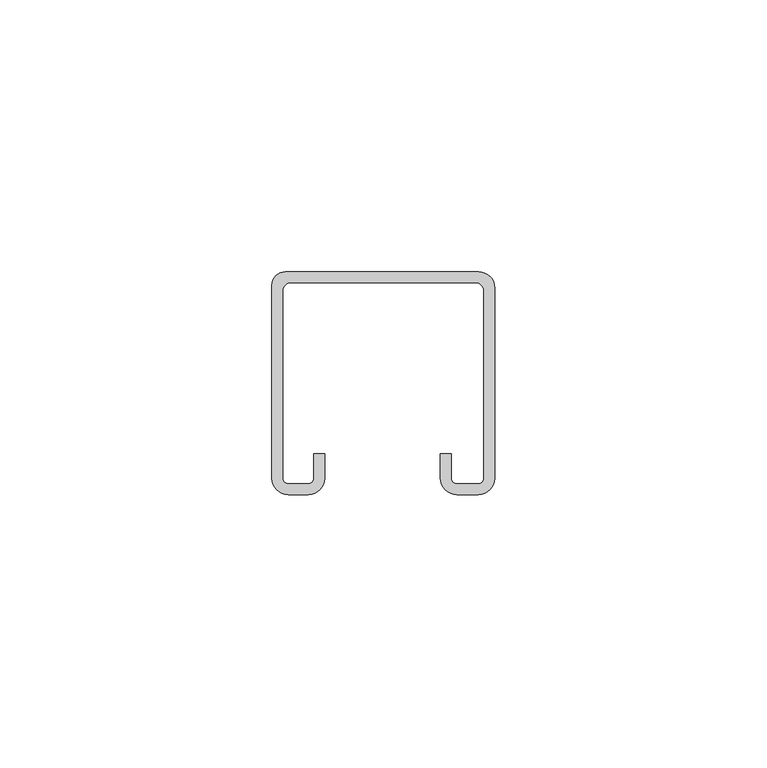
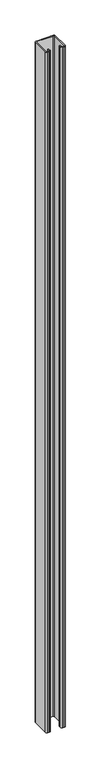
"""IFC4 building model written with IfcOpenShell, lengths in millimetres: proxy geometry, TN_Профиль монтажный : Профиль монтажный 41х41x2,0-3000."""

from ifc_helpers import new_model, si_unit, point, frame_2d, origin, origin_with_axes, place, context, project, spatial, polyline, circle_curve, trimmed, segment, composite_curve, outline, extrude, source, transform, mapped, element, save


def generic_models_c49aae80(model_context):
    return source(origin(), model_context, "Body", "SweptSolid", [
        extrude(outline(composite_curve([segment(polyline([(20.7157599, -2.9315199), (20.7157599, -38.0)]), True, "CONTINUOUS"), segment(trimmed(circle_curve(frame_2d((17.7157599, -38.0)), 3.0), [point((20.7157599, -38.0))], [point((17.7157599, -41.0))], False, "CARTESIAN"), True, "CONTINUOUS"), segment(polyline([(17.7157599, -41.0), (13.7568638, -41.0)]), True, "CONTINUOUS"), segment(trimmed(circle_curve(frame_2d((13.7568638, -37.9588961)), 3.0411039), [point((13.7568638, -41.0))], [point((10.7157599, -37.9588961))], False, "CARTESIAN"), True, "CONTINUOUS"), segment(polyline([(10.7157599, -37.9588961), (10.7157599, -33.5), (12.7157599, -33.5), (12.7157599, -38.0)]), True, "CONTINUOUS"), segment(trimmed(circle_curve(frame_2d((13.7157599, -38.0)), 1.0), [point((12.7157599, -38.0))], [point((13.7157599, -39.0))], True, "CARTESIAN"), True, "CONTINUOUS"), segment(polyline([(13.7157599, -39.0), (17.7157599, -39.0)]), True, "CONTINUOUS"), segment(trimmed(circle_curve(frame_2d((17.7157599, -38.0)), 1.0), [point((17.7157599, -39.0))], [point((18.7157599, -38.0))], True, "CARTESIAN"), True, "CONTINUOUS"), segment(polyline([(18.7157599, -38.0), (18.7157599, -3.5)]), True, "CONTINUOUS"), segment(trimmed(circle_curve(frame_2d((17.2157599, -3.5)), 1.5), [point((18.7157599, -3.5))], [point((17.2157599, -2.0))], True, "CARTESIAN"), True, "CONTINUOUS"), segment(polyline([(17.2157599, -2.0), (-16.7842401, -2.0)]), True, "CONTINUOUS"), segment(trimmed(circle_curve(frame_2d((-16.7842401, -3.5)), 1.5), [point((-16.7842401, -2.0))], [point((-18.2842401, -3.5))], True, "CARTESIAN"), True, "CONTINUOUS"), segment(polyline([(-18.2842401, -3.5), (-18.2842401, -38.0)]), True, "CONTINUOUS"), segment(trimmed(circle_curve(frame_2d((-17.2842401, -38.0)), 1.0), [point((-18.2842401, -38.0))], [point((-17.2842401, -39.0))], True, "CARTESIAN"), True, "CONTINUOUS"), segment(polyline([(-17.2842401, -39.0), (-13.5684801, -39.0)]), True, "CONTINUOUS"), segment(trimmed(circle_curve(frame_2d((-13.5684801, -38.0)), 1.0), [point((-13.5684801, -39.0))], [point((-12.5684801, -38.0))], True, "CARTESIAN"), True, "CONTINUOUS"), segment(polyline([(-12.5684801, -38.0), (-12.5684801, -33.5), (-10.5684801, -33.5), (-10.5684801, -38.0)]), True, "CONTINUOUS"), segment(trimmed(circle_curve(frame_2d((-13.5684801, -38.0)), 3.0), [point((-10.5684801, -38.0))], [point((-13.5684801, -41.0))], False, "CARTESIAN"), True, "CONTINUOUS"), segment(polyline([(-13.5684801, -41.0), (-17.2842401, -41.0)]), True, "CONTINUOUS"), segment(trimmed(circle_curve(frame_2d((-17.2842401, -38.0)), 3.0), [point((-17.2842401, -41.0))], [point((-20.2842401, -38.0))], False, "CARTESIAN"), True, "CONTINUOUS"), segment(polyline([(-20.2842401, -38.0), (-20.2842401, -2.5)]), True, "CONTINUOUS"), segment(trimmed(circle_curve(frame_2d((-17.7842401, -2.5)), 2.5), [point((-20.2842401, -2.5))], [point((-17.7842401, 0.0))], False, "CARTESIAN"), True, "CONTINUOUS"), segment(polyline([(-17.7842401, 0.0), (17.7842401, 0.0)]), True, "CONTINUOUS"), segment(trimmed(circle_curve(frame_2d((17.7842401, -2.9315199)), 2.9315199), [point((17.7842401, 0.0))], [point((20.7157599, -2.9315199))], False, "CARTESIAN"), True, "CONTINUOUS")], self_intersect=False)), origin_with_axes(), (0.0, 0.0, 1.0), 1500.0),
    ])


if __name__ == "__main__":
    model = new_model("IFC4")
    model_context = context("Model", 3, world=origin())
    ifc_project = project(units=[si_unit("LENGTHUNIT", "METRE", prefix="MILLI")], contexts=[model_context])
    site = spatial("IfcSite", under=ifc_project)
    building = spatial("IfcBuilding", under=site)
    placement = place(None, origin())
    generic_models_shape = generic_models_c49aae80(model_context)
    element("IfcBuildingElementProxy", 1, Name="TN_Профиль монтажный : Профиль монтажный 41х41x2,0-3000", ObjectType="TN_Профиль монтажный : Профиль монтажный 41х41x2,0-3000", at=placement, inside=building, context=model_context, shape_type="MappedRepresentation", body=[
        mapped(generic_models_shape, transform((0.0, 0.0, 0.0), x_axis=(1.0, 0.0, 0.0), y_axis=(0.0, 1.0, 0.0), z_axis=(0.0, 0.0, 1.0))),
    ])
    save(model, "model.ifc")

# Revit data of these elements
# Type "TN_Профиль монтажный : Профиль монтажный 41х41x2,0-3000"
#   Description = "Профиль монтажный – траверса С-образной формы предназначен для горизонтального и вертикального монтажа тяжелых инженерных систем, оборудования систем вентиляции и кондиционирования, установок электроснабжения, элементов трубопроводов, также для изготовления стенных консолей пристенного монтажа, рам оснований различного типа под оборудование. Возможно замещение на основе сконструированных модулей серийных опор ГОСТ для раскрепления технологических трубопроводов. Рекомендуется для применения в сухих, влажных помещениях и на открытом воздухе."
#   Manufacturer = "ТехноНИКОЛЬ"
#   Model = "Комплектующие к опорам"
#   URL = "https://nav.tn.ru/knowledge-base/polimernye-membrany/opory-pod-oborudovanie-na-ploskoy-krovle/?sphrase_id=266812"
#   ADSK_Обозначение = "ТехноНИКОЛЬ"
#   ADSK_Наименование краткое = "П41х41x2,0"
#   ADSK_Наименование = "Профиль монтажный 41х41x2,0-3000"
#   ADSK_Масса_Текст = ""
#   ADSK_Марка = "П41х41x2,0"
#   ADSK_Код изделия = "660816"
#   ADSK_Завод-изготовитель = "ТехноНИКОЛЬ"
#   ADSK_Единица измерения = "п.м."
#   ADSK_Группирование = "Комплектующие к опорам"
#   ADSK_URL страницы изделия = "https://nav.tn.ru/knowledge-base/polimernye-membrany/opory-pod-oborudovanie-na-ploskoy-krovle/?sphrase_id=266812"
#   ADSK_URL документации изделия = ""
#   Размер_Длина_Вводимая [instance default] = 1000 mm
#   ADSK_Размер_Длина [instance default] = 1000 mm
#   ADSK_Количество [instance default] = 1
#   Тип профиля = 1
#   Профиль монтажный 41х41x2,0 = yes
#   Профиль монтажный 41x62x2,5 = no
#   Профиль монтажный 41x124x2,5 = no
#   ADSK_Материал = TN_СтальГальванизированная_Серый
#   Default Elevation = 0
# Element 1 (IfcBuildingElementProxy, "TN_Профиль монтажный : Профиль монтажный 41х41x2,0-3000")
#   Размер_Длина_Вводимая = 1500 mm
#   ADSK_Размер_Длина = 1500 mm
#   ADSK_Количество = 1.5
#   Materials on its faces: "TN_СтальГальванизированная_Серый"
# Materials
#   "TN_СтальГальванизированная_Серый": class "Типовые", colour RGB 206 210 213, transparency 0, Cost = 0
